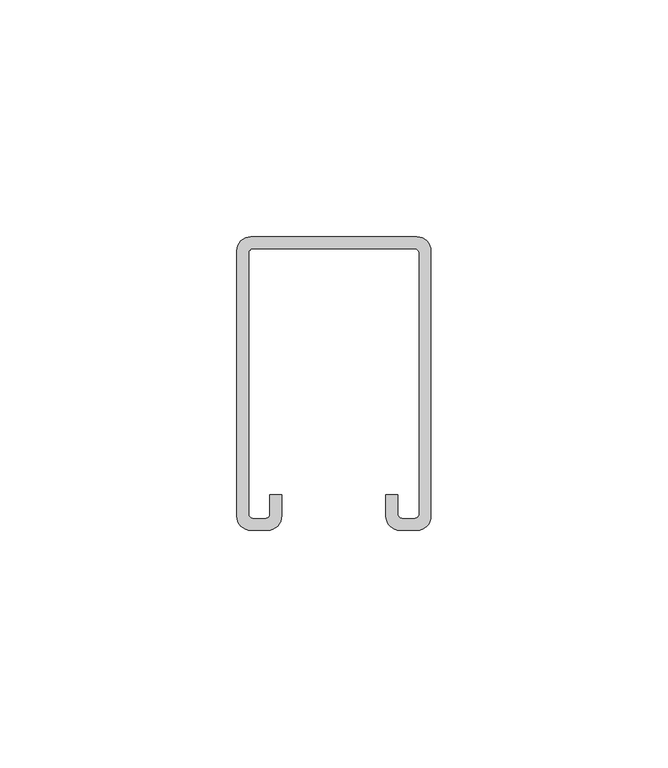
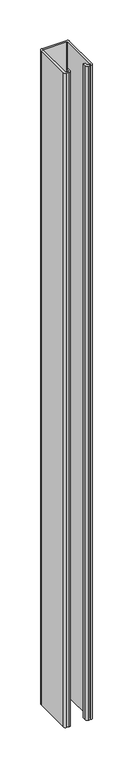
"""IFC4 building model written with IfcOpenShell, lengths in millimetres: proxy geometry, TN_Профиль монтажный : Профиль монтажный 41x62x2,5-3000."""

from ifc_helpers import new_model, si_unit, point, frame_2d, origin, origin_with_axes, place, context, project, spatial, polyline, circle_curve, trimmed, segment, composite_curve, outline, extrude, source, transform, mapped, element, save


def generic_models_c030367c(model_context):
    return source(origin(), model_context, "Body", "SweptSolid", [
        extrude(outline(composite_curve([segment(trimmed(circle_curve(frame_2d((-17.5, -3.0)), 3.0), [point((-20.5, -3.0))], [point((-17.5, 0.0))], False, "CARTESIAN"), True, "CONTINUOUS"), segment(polyline([(-17.5, 0.0), (17.5, 0.0)]), True, "CONTINUOUS"), segment(trimmed(circle_curve(frame_2d((17.5, -3.0)), 3.0), [point((17.5, 0.0))], [point((20.5, -3.0))], False, "CARTESIAN"), True, "CONTINUOUS"), segment(polyline([(20.5, -3.0), (20.5, -59.0)]), True, "CONTINUOUS"), segment(trimmed(circle_curve(frame_2d((17.5, -59.0)), 3.0), [point((20.5, -59.0))], [point((17.5, -62.0))], False, "CARTESIAN"), True, "CONTINUOUS"), segment(polyline([(17.5, -62.0), (14.0, -62.0)]), True, "CONTINUOUS"), segment(trimmed(circle_curve(frame_2d((14.0, -59.0)), 3.0), [point((14.0, -62.0))], [point((11.0, -59.0))], False, "CARTESIAN"), True, "CONTINUOUS"), segment(polyline([(11.0, -59.0), (11.0, -54.5), (13.5, -54.5), (13.5, -58.5)]), True, "CONTINUOUS"), segment(trimmed(circle_curve(frame_2d((14.5, -58.5)), 1.0), [point((13.5, -58.5))], [point((14.5, -59.5))], True, "CARTESIAN"), True, "CONTINUOUS"), segment(polyline([(14.5, -59.5), (17.0, -59.5)]), True, "CONTINUOUS"), segment(trimmed(circle_curve(frame_2d((17.0, -58.5)), 1.0), [point((17.0, -59.5))], [point((18.0, -58.5))], True, "CARTESIAN"), True, "CONTINUOUS"), segment(polyline([(18.0, -58.5), (18.0, -3.5)]), True, "CONTINUOUS"), segment(trimmed(circle_curve(frame_2d((17.0, -3.5)), 1.0), [point((18.0, -3.5))], [point((17.0, -2.5))], True, "CARTESIAN"), True, "CONTINUOUS"), segment(polyline([(17.0, -2.5), (-17.0, -2.5)]), True, "CONTINUOUS"), segment(trimmed(circle_curve(frame_2d((-17.0, -3.5)), 1.0), [point((-17.0, -2.5))], [point((-18.0, -3.5))], True, "CARTESIAN"), True, "CONTINUOUS"), segment(polyline([(-18.0, -3.5), (-18.0, -58.5)]), True, "CONTINUOUS"), segment(trimmed(circle_curve(frame_2d((-17.0, -58.5)), 1.0), [point((-18.0, -58.5))], [point((-17.0, -59.5))], True, "CARTESIAN"), True, "CONTINUOUS"), segment(polyline([(-17.0, -59.5), (-14.5, -59.5)]), True, "CONTINUOUS"), segment(trimmed(circle_curve(frame_2d((-14.5, -58.5)), 1.0), [point((-14.5, -59.5))], [point((-13.5, -58.5))], True, "CARTESIAN"), True, "CONTINUOUS"), segment(polyline([(-13.5, -58.5), (-13.5, -54.5), (-11.0, -54.5), (-11.0, -58.9588961)]), True, "CONTINUOUS"), segment(trimmed(circle_curve(frame_2d((-14.0411039, -58.9588961)), 3.0411039), [point((-11.0, -58.9588961))], [point((-14.0411039, -62.0))], False, "CARTESIAN"), True, "CONTINUOUS"), segment(polyline([(-14.0411039, -62.0), (-17.5, -62.0)]), True, "CONTINUOUS"), segment(trimmed(circle_curve(frame_2d((-17.5, -59.0)), 3.0), [point((-17.5, -62.0))], [point((-20.5, -59.0))], False, "CARTESIAN"), True, "CONTINUOUS"), segment(polyline([(-20.5, -59.0), (-20.5, -3.0)]), True, "CONTINUOUS")], self_intersect=False)), origin_with_axes(), (0.0, 0.0, 1.0), 1000.0),
    ])


if __name__ == "__main__":
    model = new_model("IFC4")
    model_context = context("Model", 3, world=origin())
    ifc_project = project(units=[si_unit("LENGTHUNIT", "METRE", prefix="MILLI")], contexts=[model_context])
    site = spatial("IfcSite", under=ifc_project)
    building = spatial("IfcBuilding", under=site)
    placement = place(None, origin())
    generic_models_shape = generic_models_c030367c(model_context)
    element("IfcBuildingElementProxy", 1, Name="TN_Профиль монтажный : Профиль монтажный 41x62x2,5-3000", ObjectType="TN_Профиль монтажный : Профиль монтажный 41x62x2,5-3000", at=placement, inside=building, context=model_context, shape_type="MappedRepresentation", body=[
        mapped(generic_models_shape, transform((0.0, 0.0, 0.0), x_axis=(1.0, 0.0, 0.0), y_axis=(0.0, 1.0, 0.0), z_axis=(0.0, 0.0, 1.0))),
    ])
    save(model, "model.ifc")

# Revit data of these elements
# Type "TN_Профиль монтажный : Профиль монтажный 41x62x2,5-3000"
#   Description = "Профиль монтажный – траверса С-образной формы предназначен для горизонтального и вертикального монтажа тяжелых инженерных систем, оборудования систем вентиляции и кондиционирования, установок электроснабжения, элементов трубопроводов, также для изготовления стенных консолей пристенного монтажа, рам оснований различного типа под оборудование. Возможно замещение на основе сконструированных модулей серийных опор ГОСТ для раскрепления технологических трубопроводов. Рекомендуется для применения в сухих, влажных помещениях и на открытом воздухе."
#   Manufacturer = "ТехноНИКОЛЬ"
#   Model = "Комплектующие к опорам"
#   URL = "https://nav.tn.ru/knowledge-base/polimernye-membrany/opory-pod-oborudovanie-na-ploskoy-krovle/?sphrase_id=266812"
#   ADSK_Обозначение = "ТехноНИКОЛЬ"
#   ADSK_Наименование краткое = "П41x62x2,5"
#   ADSK_Наименование = "Профиль монтажный 41x62x2,5-3000"
#   ADSK_Масса_Текст = ""
#   ADSK_Марка = "П41x62x2,5"
#   ADSK_Код изделия = "660817"
#   ADSK_Завод-изготовитель = "ТехноНИКОЛЬ"
#   ADSK_Единица измерения = "п.м."
#   ADSK_Группирование = "Комплектующие к опорам"
#   ADSK_URL страницы изделия = "https://nav.tn.ru/knowledge-base/polimernye-membrany/opory-pod-oborudovanie-na-ploskoy-krovle/?sphrase_id=266812"
#   ADSK_URL документации изделия = ""
#   Размер_Длина_Вводимая [instance default] = 1000 mm
#   ADSK_Размер_Длина [instance default] = 1000 mm
#   ADSK_Количество [instance default] = 1
#   Тип профиля = 1
#   Профиль монтажный 41х41x2,0 = no
#   Профиль монтажный 41x62x2,5 = yes
#   Профиль монтажный 41x124x2,5 = no
#   ADSK_Материал = TN_СтальГальванизированная_Серый
#   Default Elevation = 0
# Element 1 (IfcBuildingElementProxy, "TN_Профиль монтажный : Профиль монтажный 41x62x2,5-3000")
#   Materials on its faces: "TN_СтальГальванизированная_Серый"
# Materials
#   "TN_СтальГальванизированная_Серый": class "Типовые", colour RGB 206 210 213, transparency 0, Cost = 0
